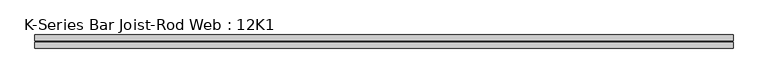
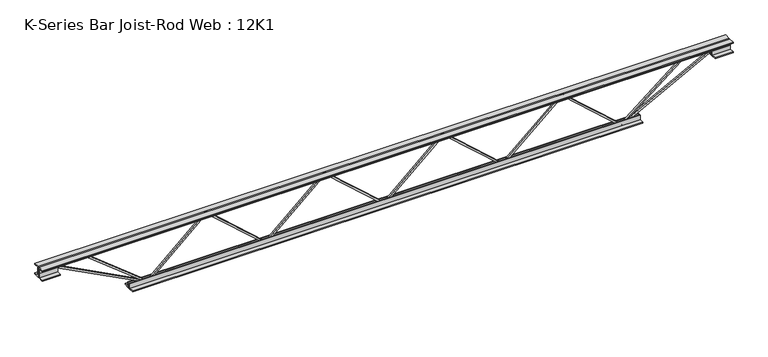
"""IFC4 building model written with IfcOpenShell, lengths in millimetres: beam geometry, K-Series Bar Joist-Rod Web : 12K1."""

import ifcopenshell
import ifcopenshell.guid

model = None  # the IFC model being written
_history = None  # IfcOwnerHistory: only IFC2X3 demands one
_inside = {}  # id of a spatial element -> (the spatial element, [elements in it])
_under = {}  # id of a project, library or spatial element -> (it, [spatial elements below it])
_declared = {}  # id of a project -> (the project, [libraries it declares])
_typed = {}  # id of a type object -> (the type object, [elements of that type])
_made_of = {}  # id of a material, layer set ... -> (it, [elements and type objects made of it])


def new_model(schema):
    """Start an empty IFC model of exactly this schema.

    Asked for "IFC4X3", IfcOpenShell would pick the latest addendum, in which some entities
    have other attributes; the version numbers below select the first issue.
    IFC2X3 requires an IfcOwnerHistory on every rooted entity: one is made here for all.
    """
    global model, _history
    if schema == "IFC4X3":
        model = ifcopenshell.file(schema_version=(4, 3, 0, 0))
    else:
        model = ifcopenshell.file(schema=schema)
    _inside.clear()
    _under.clear()
    _declared.clear()
    _typed.clear()
    _made_of.clear()
    _history = None
    if model.schema == "IFC2X3":
        org = make("IfcOrganization", Name="unknown")
        user = make(
            "IfcPersonAndOrganization",
            ThePerson=make("IfcPerson", FamilyName="unknown"),
            TheOrganization=org,
        )
        app = make(
            "IfcApplication",
            ApplicationDeveloper=org,
            Version="unknown",
            ApplicationFullName="unknown",
            ApplicationIdentifier="unknown",
        )
        _history = make(
            "IfcOwnerHistory",
            OwningUser=user,
            OwningApplication=app,
            ChangeAction="ADDED",
            CreationDate=0,
        )
    return model


def make(cls, **values):
    """One entity of the class cls with the attributes given. An attribute that is None is left unset."""
    return model.create_entity(
        cls, **{name: value for name, value in values.items() if value is not None}
    )


def rooted(cls, **values):
    """An entity with a GlobalId (a new one), such as an element, a storey or a relation."""
    return make(cls, GlobalId=ifcopenshell.guid.new(), OwnerHistory=_history, **values)


def si_unit(unit_type, name, prefix=None):
    """IfcSIUnit, for example si_unit("LENGTHUNIT", "METRE", prefix="MILLI")."""
    return make("IfcSIUnit", UnitType=unit_type, Prefix=prefix, Name=name)


def assignment(units):
    """IfcUnitAssignment: the units of a project."""
    return None if units is None else make("IfcUnitAssignment", Units=units)


def point(xyz):
    """IfcCartesianPoint."""
    return None if xyz is None else make("IfcCartesianPoint", Coordinates=xyz)


def direction(xyz):
    """IfcDirection."""
    return None if xyz is None else make("IfcDirection", DirectionRatios=xyz)


def frame(location, z_axis=None, x_axis=None):
    """IfcAxis2Placement3D, a coordinate frame: its origin and axes. An axis left out is left unset."""
    return make(
        "IfcAxis2Placement3D",
        Location=point(location),
        Axis=direction(z_axis),
        RefDirection=direction(x_axis),
    )


def origin():
    """The frame at (0, 0, 0) with its axes left unset."""
    return frame((0.0, 0.0, 0.0))


def place(relative_to, where):
    """IfcLocalPlacement: puts the frame where relative to a parent placement (None: the world)."""
    return make(
        "IfcLocalPlacement", PlacementRelTo=relative_to, RelativePlacement=where
    )


def context(
    kind, dimensions, precision=None, world=None, true_north=None, identifier=None
):
    """IfcGeometricRepresentationContext, for example the 3D "Model" context."""
    return make(
        "IfcGeometricRepresentationContext",
        ContextIdentifier=identifier,
        ContextType=kind,
        CoordinateSpaceDimension=dimensions,
        Precision=precision,
        WorldCoordinateSystem=world,
        TrueNorth=true_north,
    )


def project(units=None, contexts=None):
    """IfcProject with its units and contexts."""
    return rooted(
        "IfcProject",
        Name="project",
        RepresentationContexts=contexts,
        UnitsInContext=assignment(units),
    )


def spatial(cls, under=None, at=None, **own):
    """A site, building, storey or space (cls), placed at a placement, below another one or the project."""
    s = rooted(cls, ObjectPlacement=at, **own)
    if under is not None:
        _under.setdefault(under.id(), (under, []))[1].append(s)
    return s


def polyline(points):
    """IfcPolyline through the points."""
    return make("IfcPolyline", Points=[point(p) for p in points])


def outline(outer, holes=None, kind="AREA"):
    """IfcArbitraryClosedProfileDef: a profile drawn as a closed curve; with holes, ...WithVoids."""
    if holes is None:
        return make("IfcArbitraryClosedProfileDef", ProfileType=kind, OuterCurve=outer)
    return make(
        "IfcArbitraryProfileDefWithVoids",
        ProfileType=kind,
        OuterCurve=outer,
        InnerCurves=holes,
    )


def extrude(swept, where, along, depth):
    """IfcExtrudedAreaSolid: the profile swept, set in the frame where, extruded along a direction by depth."""
    return make(
        "IfcExtrudedAreaSolid",
        SweptArea=swept,
        Position=where,
        ExtrudedDirection=direction(along),
        Depth=depth,
    )


def shape(context_of_items, identifier, shape_type, items):
    """IfcShapeRepresentation: the items that make up one representation, for example the "Body"."""
    return make(
        "IfcShapeRepresentation",
        ContextOfItems=context_of_items,
        RepresentationIdentifier=identifier,
        RepresentationType=shape_type,
        Items=items,
    )


def source(mapping_origin, context_of_items, identifier, shape_type, items):
    """IfcRepresentationMap: a shape defined once, which mapped items show again and again."""
    return make(
        "IfcRepresentationMap",
        MappingOrigin=mapping_origin,
        MappedRepresentation=shape(context_of_items, identifier, shape_type, items),
    )


def transform(
    local_origin,
    x_axis=None,
    y_axis=None,
    z_axis=None,
    scale=None,
    scale2=None,
    scale3=None,
    uniform=True,
):
    """IfcCartesianTransformationOperator3D, or its non-uniform kind. x_axis, y_axis, z_axis: its Axis1, 2, 3."""
    if uniform:
        return make(
            "IfcCartesianTransformationOperator3D",
            Axis1=direction(x_axis),
            Axis2=direction(y_axis),
            LocalOrigin=point(local_origin),
            Scale=scale,
            Axis3=direction(z_axis),
        )
    return make(
        "IfcCartesianTransformationOperator3DnonUniform",
        Axis1=direction(x_axis),
        Axis2=direction(y_axis),
        LocalOrigin=point(local_origin),
        Scale=scale,
        Axis3=direction(z_axis),
        Scale2=scale2,
        Scale3=scale3,
    )


def mapped(mapping_source, mapping_target):
    """IfcMappedItem: shows the shape of a source again, moved by a transform."""
    return make(
        "IfcMappedItem", MappingSource=mapping_source, MappingTarget=mapping_target
    )


def made_of(thing, what):
    """Note that an element or type object is made of a material, layer set ...; save() writes the relation."""
    if what is not None:
        _made_of.setdefault(what.id(), (what, []))[1].append(thing)
    return thing


def element(
    cls,
    number,
    at=None,
    inside=None,
    cuts=None,
    type_object=None,
    material=None,
    context=None,
    identifier="Body",
    shape_type=None,
    held_by="IfcProductDefinitionShape",
    body=None,
    shapes=None,
    **own,
):
    """One element of the class cls, such as IfcWall. Its Tag is "e" and its number.

    at: its placement. inside: the storey or other place that contains it. cuts: it is an
    opening in that element (IfcRelVoidsElement). A single representation is given by context,
    identifier, shape_type and body (its items); several are given by shapes. held_by: the class
    of the entity that holds the representations. save() writes the other relations.
    """
    e = rooted(cls, Tag="e%d" % number, ObjectPlacement=at, **own)
    if body is not None:
        shapes = [shape(context, identifier, shape_type, body)]
    if shapes is not None:
        e.Representation = make(held_by, Representations=shapes)
    if inside is not None:
        _inside.setdefault(inside.id(), (inside, []))[1].append(e)
    if cuts is not None:
        rooted(
            "IfcRelVoidsElement", RelatingBuildingElement=cuts, RelatedOpeningElement=e
        )
    if type_object is not None:
        _typed.setdefault(type_object.id(), (type_object, []))[1].append(e)
    return made_of(e, material)


def aggregate(whole, parts):
    """IfcRelAggregates: a whole, such as a stair, and the parts it consists of."""
    return rooted("IfcRelAggregates", RelatingObject=whole, RelatedObjects=parts)


def save(model, path):
    """Write the relations noted so far, then the file.

    IfcRelAggregates (storeys below a building ...), IfcRelContainedInSpatialStructure (elements
    in a storey), IfcRelDefinesByType, IfcRelAssociatesMaterial and IfcRelDeclares: one each for
    every whole, place, type object, material and project.
    """
    for whole, parts in _under.values():
        aggregate(whole, parts)
    for where, things in _inside.values():
        rooted(
            "IfcRelContainedInSpatialStructure",
            RelatedElements=things,
            RelatingStructure=where,
        )
    for kind, things in _typed.values():
        rooted("IfcRelDefinesByType", RelatedObjects=things, RelatingType=kind)
    for what, things in _made_of.values():
        rooted("IfcRelAssociatesMaterial", RelatedObjects=things, RelatingMaterial=what)
    for by, libraries in _declared.values():
        rooted("IfcRelDeclares", RelatingContext=by, RelatedDefinitions=libraries)
    model.write(path)


def k_series_bar_joist_rod_web_12k1_0543d242(model_context):
    return source(origin(), model_context, "Body", "SweptSolid", [
        extrude(outline(polyline([(-141.2875, 0.0), (-150.8125, 0.0), (-150.8125, 4.9889734), (141.2875, 332.8077234), (141.2875, 335.5297766), (-150.8125, 663.3485266), (-150.8125, 668.3375), (-141.2875, 668.3375), (-141.2875, 666.9764734), (150.8125, 339.1577234), (150.8125, 329.1797766), (-141.2875, 1.3610266), (-141.2875, 0.0)])), frame((0.0, -4.7625, 0.0), z_axis=(0.0, 1.0, 0.0), x_axis=(0.0, 0.0, 1.0)), (0.0, 0.0, 1.0), 9.525),
        extrude(outline(polyline([(-141.2875, -668.3375), (-150.8125, -668.3375), (-150.8125, -663.3485266), (141.2875, -335.5297766), (141.2875, -332.8077234), (-150.8125, -4.9889734), (-150.8125, 0.0), (-141.2875, 0.0), (-141.2875, -1.3610266), (150.8125, -329.1797766), (150.8125, -339.1577234), (-141.2875, -666.9764734), (-141.2875, -668.3375)])), frame((0.0, -4.7625, 0.0), z_axis=(0.0, 1.0, 0.0), x_axis=(0.0, 0.0, 1.0)), (0.0, 0.0, 1.0), 9.525),
        extrude(outline(polyline([(-141.2875, 668.3375), (-150.8125, 668.3375), (-150.8125, 673.3264734), (141.2875, 1001.1452234), (141.2875, 1003.8672766), (-150.8125, 1331.6860266), (-150.8125, 1336.675), (-141.2875, 1336.675), (-141.2875, 1335.3139734), (150.8125, 1007.4952234), (150.8125, 997.5172766), (-141.2875, 669.6985266), (-141.2875, 668.3375)])), frame((0.0, -4.7625, 0.0), z_axis=(0.0, 1.0, 0.0), x_axis=(0.0, 0.0, 1.0)), (0.0, 0.0, 1.0), 9.525),
        extrude(outline(polyline([(-141.2875, -1336.675), (-150.8125, -1336.675), (-150.8125, -1331.6860266), (141.2875, -1003.8672766), (141.2875, -1001.1452234), (-150.8125, -673.3264734), (-150.8125, -668.3375), (-141.2875, -668.3375), (-141.2875, -669.6985266), (150.8125, -997.5172766), (150.8125, -1007.4952234), (-141.2875, -1335.3139734), (-141.2875, -1336.675)])), frame((0.0, -4.7625, 0.0), z_axis=(0.0, 1.0, 0.0), x_axis=(0.0, 0.0, 1.0)), (0.0, 0.0, 1.0), 9.525),
        extrude(outline(polyline([(4.7625, 152.4), (36.5125, 152.4), (36.5125, 146.05), (11.1125, 146.05), (11.1125, 120.65), (4.7625, 120.65), (4.7625, 152.4)])), frame((-1946.275, 0.0, 0.0), z_axis=(1.0, 0.0, 0.0), x_axis=(0.0, 1.0, 0.0)), (0.0, 0.0, 1.0), 3892.55),
        extrude(outline(polyline([(-4.7625, 152.4), (-4.7625, 120.65), (-11.1125, 120.65), (-11.1125, 146.05), (-36.5125, 146.05), (-36.5125, 152.4), (-4.7625, 152.4)])), frame((-1946.275, 0.0, 0.0), z_axis=(1.0, 0.0, 0.0), x_axis=(0.0, 1.0, 0.0)), (0.0, 0.0, 1.0), 3892.55),
        extrude(outline(polyline([(-4.7625, 88.9), (-36.5125, 88.9), (-36.5125, 95.25), (-11.1125, 95.25), (-11.1125, 120.65), (-4.7625, 120.65), (-4.7625, 88.9)])), frame((-1946.275, 0.0, 0.0), z_axis=(1.0, 0.0, 0.0), x_axis=(0.0, 1.0, 0.0)), (0.0, 0.0, 1.0), 101.6),
        extrude(outline(polyline([(36.5125, 88.9), (4.7625, 88.9), (4.7625, 120.65), (11.1125, 120.65), (11.1125, 95.25), (36.5125, 95.25), (36.5125, 88.9)])), frame((-1946.275, 0.0, 0.0), z_axis=(1.0, 0.0, 0.0), x_axis=(0.0, 1.0, 0.0)), (0.0, 0.0, 1.0), 101.6),
        extrude(outline(polyline([(4.7625, 88.9), (4.7625, 120.65), (11.1125, 120.65), (11.1125, 95.25), (36.5125, 95.25), (36.5125, 88.9), (4.7625, 88.9)])), frame((1844.675, 0.0, 0.0), z_axis=(1.0, 0.0, 0.0), x_axis=(0.0, 1.0, 0.0)), (0.0, 0.0, 1.0), 101.6),
        extrude(outline(polyline([(-4.7625, 88.9), (-36.5125, 88.9), (-36.5125, 95.25), (-11.1125, 95.25), (-11.1125, 120.65), (-4.7625, 120.65), (-4.7625, 88.9)])), frame((1844.675, 0.0, 0.0), z_axis=(1.0, 0.0, 0.0), x_axis=(0.0, 1.0, 0.0)), (0.0, 0.0, 1.0), 101.6),
        extrude(outline(polyline([(4.7625, -152.4), (4.7625, -120.65), (11.1125, -120.65), (11.1125, -146.05), (36.5125, -146.05), (36.5125, -152.4), (4.7625, -152.4)])), frame((-1438.275, 0.0, 0.0), z_axis=(1.0, 0.0, 0.0), x_axis=(0.0, 1.0, 0.0)), (0.0, 0.0, 1.0), 2876.55),
        extrude(outline(polyline([(-4.7625, -152.4), (-36.5125, -152.4), (-36.5125, -146.05), (-11.1125, -146.05), (-11.1125, -120.65), (-4.7625, -120.65), (-4.7625, -152.4)])), frame((-1438.275, 0.0, 0.0), z_axis=(1.0, 0.0, 0.0), x_axis=(0.0, 1.0, 0.0)), (0.0, 0.0, 1.0), 2876.55),
        extrude(outline(polyline([(0.0, -9.525), (0.0, 0.0), (573.7533355, 0.0), (573.7533355, -9.525), (0.0, -9.525)])), frame((-1846.8887714, 4.7625, 116.4332925), z_axis=(0.46483389898951394, 0.0, 0.8853979028381569), x_axis=(0.8853979028381569, 0.0, -0.46483389898951394)), (0.0, 0.0, 1.0), 9.525),
        extrude(outline(polyline([(0.0, -9.525), (0.0, 0.0), (427.5484107, 0.0), (427.5484107, -9.525), (0.0, -9.525)])), frame((-1673.8145452, 4.7625, 116.9276644), z_axis=(0.6237890104058852, 0.0, 0.7815927779200922), x_axis=(0.7815927779200922, 0.0, -0.6237890104058852)), (0.0, 0.0, 1.0), 9.525),
        extrude(outline(polyline([(0.0, -9.525), (0.0, 0.0), (573.7533355, 0.0), (573.7533355, -9.525), (0.0, -9.525)])), frame((1846.8887714, -4.7625, 116.4332925), z_axis=(-0.4648338989894953, 0.0, 0.8853979028381667), x_axis=(-0.8853979028381667, 0.0, -0.4648338989894953)), (0.0, 0.0, 1.0), 9.525),
        extrude(outline(polyline([(0.0, -9.525), (0.0, 0.0), (427.5484107, 0.0), (427.5484107, -9.525), (0.0, -9.525)])), frame((1673.8145452, -4.7625, 116.9276644), z_axis=(-0.6237890104058799, 0.0, 0.7815927779200965), x_axis=(-0.7815927779200965, 0.0, -0.6237890104058799)), (0.0, 0.0, 1.0), 9.525),
    ])


if __name__ == "__main__":
    model = new_model("IFC4")
    model_context = context("Model", 3, world=origin())
    ifc_project = project(units=[si_unit("LENGTHUNIT", "METRE", prefix="MILLI")], contexts=[model_context])
    site = spatial("IfcSite", under=ifc_project)
    building = spatial("IfcBuilding", under=site)
    placement = place(None, origin())
    k_series_bar_joist_rod_web_12k1_shape = k_series_bar_joist_rod_web_12k1_0543d242(model_context)
    element("IfcBeam", 1, ObjectType="K-Series Bar Joist-Rod Web : 12K1", at=placement, inside=building, context=model_context, shape_type="MappedRepresentation", body=[
        mapped(k_series_bar_joist_rod_web_12k1_shape, transform((0.0, 0.0, 0.0), x_axis=(1.0, 0.0, 0.0), y_axis=(0.0, 1.0, 0.0), z_axis=(0.0, 0.0, 1.0))),
    ])
    save(model, "model.ifc")

# Revit data of these elements
# Type "K-Series Bar Joist-Rod Web : 12K1"
#   Assembly Code = "B1010350"
#   Wt = 5
#   Web Thickness = 0' - 0 3/8"
#   Start Offset [instance default] = 0' - 0"
#   Start Extension [instance default] = 0' - 0"
#   Seat Length = 0' - 4"
#   Seat Depth = 0' - 2 1/2"
#   PanelArrayLength [instance default] = 20' - 0"
#   Panel [instance default] = 2' - 0"
#   End Offset [instance default] = 0' - 0"
#   End Extension [instance default] = 0' - 0"
#   End Panel = 2' - 0"
#   Cord Leg = 0' - 1 1/4"
#   Chord Thickness = 0' - 0 1/4"
#   Length [instance default] = 24' - 0"
#   Depth = 1' - 0"
#   PanelArrayNum [instance default] = 10
#   Structural Material = none
# Element 1 (IfcBeam, "K-Series Bar Joist-Rod Web : 12K1")
#   PanelArrayLength = 8' - 9 1/4"
#   Panel = 2' - 2 5/16"
#   PanelArrayNum = 4
